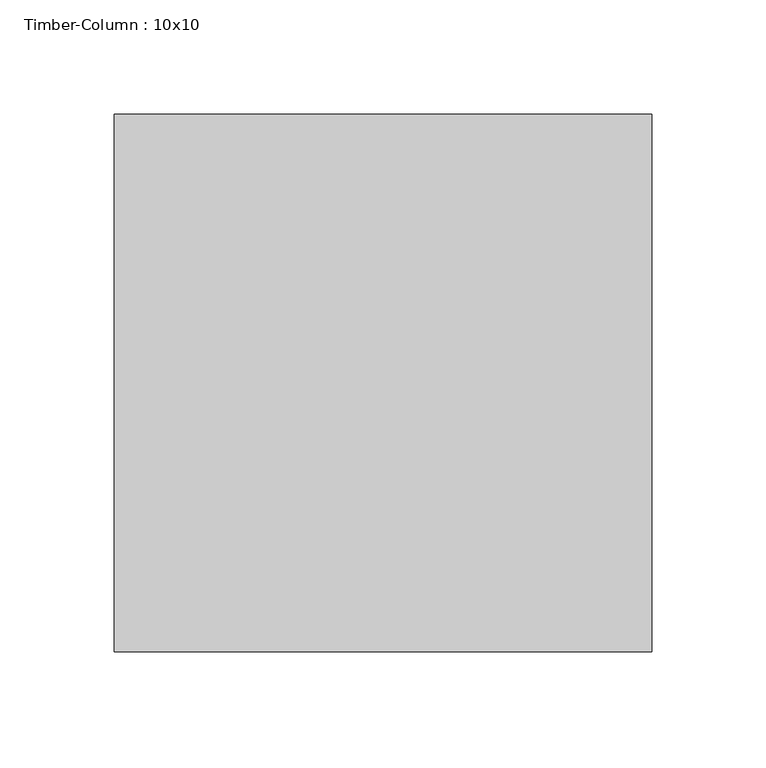
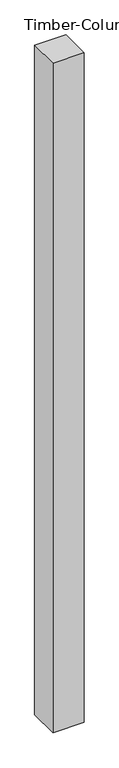
"""IFC4 building model written with IfcOpenShell, lengths in millimetres: column geometry, Timber-Column : 10x10."""

import ifcopenshell
import ifcopenshell.guid

model = None  # the IFC model being written
_history = None  # IfcOwnerHistory: only IFC2X3 demands one
_inside = {}  # id of a spatial element -> (the spatial element, [elements in it])
_under = {}  # id of a project, library or spatial element -> (it, [spatial elements below it])
_declared = {}  # id of a project -> (the project, [libraries it declares])
_typed = {}  # id of a type object -> (the type object, [elements of that type])
_made_of = {}  # id of a material, layer set ... -> (it, [elements and type objects made of it])


def new_model(schema):
    """Start an empty IFC model of exactly this schema.

    Asked for "IFC4X3", IfcOpenShell would pick the latest addendum, in which some entities
    have other attributes; the version numbers below select the first issue.
    IFC2X3 requires an IfcOwnerHistory on every rooted entity: one is made here for all.
    """
    global model, _history
    if schema == "IFC4X3":
        model = ifcopenshell.file(schema_version=(4, 3, 0, 0))
    else:
        model = ifcopenshell.file(schema=schema)
    _inside.clear()
    _under.clear()
    _declared.clear()
    _typed.clear()
    _made_of.clear()
    _history = None
    if model.schema == "IFC2X3":
        org = make("IfcOrganization", Name="unknown")
        user = make(
            "IfcPersonAndOrganization",
            ThePerson=make("IfcPerson", FamilyName="unknown"),
            TheOrganization=org,
        )
        app = make(
            "IfcApplication",
            ApplicationDeveloper=org,
            Version="unknown",
            ApplicationFullName="unknown",
            ApplicationIdentifier="unknown",
        )
        _history = make(
            "IfcOwnerHistory",
            OwningUser=user,
            OwningApplication=app,
            ChangeAction="ADDED",
            CreationDate=0,
        )
    return model


def make(cls, **values):
    """One entity of the class cls with the attributes given. An attribute that is None is left unset."""
    return model.create_entity(
        cls, **{name: value for name, value in values.items() if value is not None}
    )


def rooted(cls, **values):
    """An entity with a GlobalId (a new one), such as an element, a storey or a relation."""
    return make(cls, GlobalId=ifcopenshell.guid.new(), OwnerHistory=_history, **values)


def si_unit(unit_type, name, prefix=None):
    """IfcSIUnit, for example si_unit("LENGTHUNIT", "METRE", prefix="MILLI")."""
    return make("IfcSIUnit", UnitType=unit_type, Prefix=prefix, Name=name)


def assignment(units):
    """IfcUnitAssignment: the units of a project."""
    return None if units is None else make("IfcUnitAssignment", Units=units)


def point(xyz):
    """IfcCartesianPoint."""
    return None if xyz is None else make("IfcCartesianPoint", Coordinates=xyz)


def direction(xyz):
    """IfcDirection."""
    return None if xyz is None else make("IfcDirection", DirectionRatios=xyz)


def frame(location, z_axis=None, x_axis=None):
    """IfcAxis2Placement3D, a coordinate frame: its origin and axes. An axis left out is left unset."""
    return make(
        "IfcAxis2Placement3D",
        Location=point(location),
        Axis=direction(z_axis),
        RefDirection=direction(x_axis),
    )


def origin():
    """The frame at (0, 0, 0) with its axes left unset."""
    return frame((0.0, 0.0, 0.0))


def origin_with_axes():
    """The frame at (0, 0, 0) with the z axis (0, 0, 1) and the x axis (1, 0, 0) written out."""
    return frame((0.0, 0.0, 0.0), z_axis=(0.0, 0.0, 1.0), x_axis=(1.0, 0.0, 0.0))


def place(relative_to, where):
    """IfcLocalPlacement: puts the frame where relative to a parent placement (None: the world)."""
    return make(
        "IfcLocalPlacement", PlacementRelTo=relative_to, RelativePlacement=where
    )


def context(
    kind, dimensions, precision=None, world=None, true_north=None, identifier=None
):
    """IfcGeometricRepresentationContext, for example the 3D "Model" context."""
    return make(
        "IfcGeometricRepresentationContext",
        ContextIdentifier=identifier,
        ContextType=kind,
        CoordinateSpaceDimension=dimensions,
        Precision=precision,
        WorldCoordinateSystem=world,
        TrueNorth=true_north,
    )


def project(units=None, contexts=None):
    """IfcProject with its units and contexts."""
    return rooted(
        "IfcProject",
        Name="project",
        RepresentationContexts=contexts,
        UnitsInContext=assignment(units),
    )


def spatial(cls, under=None, at=None, **own):
    """A site, building, storey or space (cls), placed at a placement, below another one or the project."""
    s = rooted(cls, ObjectPlacement=at, **own)
    if under is not None:
        _under.setdefault(under.id(), (under, []))[1].append(s)
    return s


def polyline(points):
    """IfcPolyline through the points."""
    return make("IfcPolyline", Points=[point(p) for p in points])


def outline(outer, holes=None, kind="AREA"):
    """IfcArbitraryClosedProfileDef: a profile drawn as a closed curve; with holes, ...WithVoids."""
    if holes is None:
        return make("IfcArbitraryClosedProfileDef", ProfileType=kind, OuterCurve=outer)
    return make(
        "IfcArbitraryProfileDefWithVoids",
        ProfileType=kind,
        OuterCurve=outer,
        InnerCurves=holes,
    )


def extrude(swept, where, along, depth):
    """IfcExtrudedAreaSolid: the profile swept, set in the frame where, extruded along a direction by depth."""
    return make(
        "IfcExtrudedAreaSolid",
        SweptArea=swept,
        Position=where,
        ExtrudedDirection=direction(along),
        Depth=depth,
    )


def shape(context_of_items, identifier, shape_type, items):
    """IfcShapeRepresentation: the items that make up one representation, for example the "Body"."""
    return make(
        "IfcShapeRepresentation",
        ContextOfItems=context_of_items,
        RepresentationIdentifier=identifier,
        RepresentationType=shape_type,
        Items=items,
    )


def source(mapping_origin, context_of_items, identifier, shape_type, items):
    """IfcRepresentationMap: a shape defined once, which mapped items show again and again."""
    return make(
        "IfcRepresentationMap",
        MappingOrigin=mapping_origin,
        MappedRepresentation=shape(context_of_items, identifier, shape_type, items),
    )


def transform(
    local_origin,
    x_axis=None,
    y_axis=None,
    z_axis=None,
    scale=None,
    scale2=None,
    scale3=None,
    uniform=True,
):
    """IfcCartesianTransformationOperator3D, or its non-uniform kind. x_axis, y_axis, z_axis: its Axis1, 2, 3."""
    if uniform:
        return make(
            "IfcCartesianTransformationOperator3D",
            Axis1=direction(x_axis),
            Axis2=direction(y_axis),
            LocalOrigin=point(local_origin),
            Scale=scale,
            Axis3=direction(z_axis),
        )
    return make(
        "IfcCartesianTransformationOperator3DnonUniform",
        Axis1=direction(x_axis),
        Axis2=direction(y_axis),
        LocalOrigin=point(local_origin),
        Scale=scale,
        Axis3=direction(z_axis),
        Scale2=scale2,
        Scale3=scale3,
    )


def mapped(mapping_source, mapping_target):
    """IfcMappedItem: shows the shape of a source again, moved by a transform."""
    return make(
        "IfcMappedItem", MappingSource=mapping_source, MappingTarget=mapping_target
    )


def made_of(thing, what):
    """Note that an element or type object is made of a material, layer set ...; save() writes the relation."""
    if what is not None:
        _made_of.setdefault(what.id(), (what, []))[1].append(thing)
    return thing


def element(
    cls,
    number,
    at=None,
    inside=None,
    cuts=None,
    type_object=None,
    material=None,
    context=None,
    identifier="Body",
    shape_type=None,
    held_by="IfcProductDefinitionShape",
    body=None,
    shapes=None,
    **own,
):
    """One element of the class cls, such as IfcWall. Its Tag is "e" and its number.

    at: its placement. inside: the storey or other place that contains it. cuts: it is an
    opening in that element (IfcRelVoidsElement). A single representation is given by context,
    identifier, shape_type and body (its items); several are given by shapes. held_by: the class
    of the entity that holds the representations. save() writes the other relations.
    """
    e = rooted(cls, Tag="e%d" % number, ObjectPlacement=at, **own)
    if body is not None:
        shapes = [shape(context, identifier, shape_type, body)]
    if shapes is not None:
        e.Representation = make(held_by, Representations=shapes)
    if inside is not None:
        _inside.setdefault(inside.id(), (inside, []))[1].append(e)
    if cuts is not None:
        rooted(
            "IfcRelVoidsElement", RelatingBuildingElement=cuts, RelatedOpeningElement=e
        )
    if type_object is not None:
        _typed.setdefault(type_object.id(), (type_object, []))[1].append(e)
    return made_of(e, material)


def aggregate(whole, parts):
    """IfcRelAggregates: a whole, such as a stair, and the parts it consists of."""
    return rooted("IfcRelAggregates", RelatingObject=whole, RelatedObjects=parts)


def save(model, path):
    """Write the relations noted so far, then the file.

    IfcRelAggregates (storeys below a building ...), IfcRelContainedInSpatialStructure (elements
    in a storey), IfcRelDefinesByType, IfcRelAssociatesMaterial and IfcRelDeclares: one each for
    every whole, place, type object, material and project.
    """
    for whole, parts in _under.values():
        aggregate(whole, parts)
    for where, things in _inside.values():
        rooted(
            "IfcRelContainedInSpatialStructure",
            RelatedElements=things,
            RelatingStructure=where,
        )
    for kind, things in _typed.values():
        rooted("IfcRelDefinesByType", RelatedObjects=things, RelatingType=kind)
    for what, things in _made_of.values():
        rooted("IfcRelAssociatesMaterial", RelatedObjects=things, RelatingMaterial=what)
    for by, libraries in _declared.values():
        rooted("IfcRelDeclares", RelatingContext=by, RelatedDefinitions=libraries)
    model.write(path)


def timber_column_10x10_6788f727(model_context):
    return source(origin(), model_context, "Body", "SweptSolid", [
        extrude(outline(polyline([(117.475, 117.475), (117.475, -117.475), (-117.475, -117.475), (-117.475, 117.475), (117.475, 117.475)])), origin_with_axes(), (0.0, 0.0, 1.0), 5308.6),
    ])


if __name__ == "__main__":
    model = new_model("IFC4")
    model_context = context("Model", 3, world=origin())
    ifc_project = project(units=[si_unit("LENGTHUNIT", "METRE", prefix="MILLI")], contexts=[model_context])
    site = spatial("IfcSite", under=ifc_project)
    building = spatial("IfcBuilding", under=site)
    placement = place(None, origin())
    timber_column_10x10_shape = timber_column_10x10_6788f727(model_context)
    element("IfcColumn", 1, ObjectType="Timber-Column : 10x10", at=placement, inside=building, context=model_context, shape_type="MappedRepresentation", body=[
        mapped(timber_column_10x10_shape, transform((0.0, 0.0, 0.0), x_axis=(1.0, 0.0, 0.0), y_axis=(0.0, 1.0, 0.0), z_axis=(0.0, 0.0, 1.0))),
    ])
    save(model, "model.ifc")

# Revit data of these elements
# Type "Timber-Column : 10x10"
#   Assembly Code = "B10"
#   A = 0.210069 SF
#   b = 0' - 9 1/4"
#   d = 0' - 9 1/4"
#   Structural Material = (4) CHARRED SISTERED 2X10s AT BEAM
# Element 1 (IfcColumn, "Timber-Column : 10x10")
#   Materials on its faces: "(4) CHARRED SISTERED 2X10s AT BEAM"
# Materials
#   "(4) CHARRED SISTERED 2X10s AT BEAM": class "Wood", colour RGB 144 144 144, transparency 0, Description = "Pinus Echinata", Cost = 0
